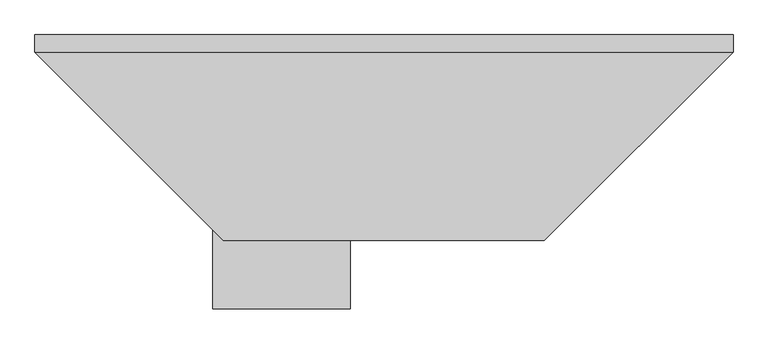
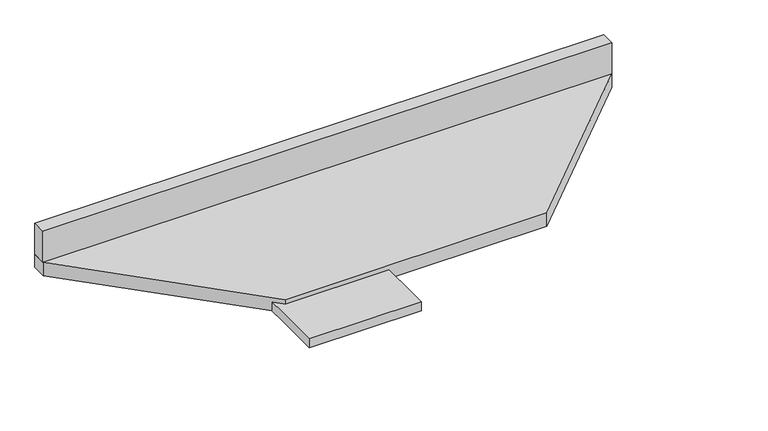
"""IFC4 building model written with IfcOpenShell, lengths in millimetres: proxy geometry, CT020 - Countertop, SS, No Opening - Angled : CT020 - Countertop, SS, No Opening - Angled."""

import ifcopenshell
import ifcopenshell.guid

model = None  # the IFC model being written
_history = None  # IfcOwnerHistory: only IFC2X3 demands one
_inside = {}  # id of a spatial element -> (the spatial element, [elements in it])
_under = {}  # id of a project, library or spatial element -> (it, [spatial elements below it])
_declared = {}  # id of a project -> (the project, [libraries it declares])
_typed = {}  # id of a type object -> (the type object, [elements of that type])
_made_of = {}  # id of a material, layer set ... -> (it, [elements and type objects made of it])


def new_model(schema):
    """Start an empty IFC model of exactly this schema.

    Asked for "IFC4X3", IfcOpenShell would pick the latest addendum, in which some entities
    have other attributes; the version numbers below select the first issue.
    IFC2X3 requires an IfcOwnerHistory on every rooted entity: one is made here for all.
    """
    global model, _history
    if schema == "IFC4X3":
        model = ifcopenshell.file(schema_version=(4, 3, 0, 0))
    else:
        model = ifcopenshell.file(schema=schema)
    _inside.clear()
    _under.clear()
    _declared.clear()
    _typed.clear()
    _made_of.clear()
    _history = None
    if model.schema == "IFC2X3":
        org = make("IfcOrganization", Name="unknown")
        user = make(
            "IfcPersonAndOrganization",
            ThePerson=make("IfcPerson", FamilyName="unknown"),
            TheOrganization=org,
        )
        app = make(
            "IfcApplication",
            ApplicationDeveloper=org,
            Version="unknown",
            ApplicationFullName="unknown",
            ApplicationIdentifier="unknown",
        )
        _history = make(
            "IfcOwnerHistory",
            OwningUser=user,
            OwningApplication=app,
            ChangeAction="ADDED",
            CreationDate=0,
        )
    return model


def make(cls, **values):
    """One entity of the class cls with the attributes given. An attribute that is None is left unset."""
    return model.create_entity(
        cls, **{name: value for name, value in values.items() if value is not None}
    )


def rooted(cls, **values):
    """An entity with a GlobalId (a new one), such as an element, a storey or a relation."""
    return make(cls, GlobalId=ifcopenshell.guid.new(), OwnerHistory=_history, **values)


def si_unit(unit_type, name, prefix=None):
    """IfcSIUnit, for example si_unit("LENGTHUNIT", "METRE", prefix="MILLI")."""
    return make("IfcSIUnit", UnitType=unit_type, Prefix=prefix, Name=name)


def assignment(units):
    """IfcUnitAssignment: the units of a project."""
    return None if units is None else make("IfcUnitAssignment", Units=units)


def point(xyz):
    """IfcCartesianPoint."""
    return None if xyz is None else make("IfcCartesianPoint", Coordinates=xyz)


def direction(xyz):
    """IfcDirection."""
    return None if xyz is None else make("IfcDirection", DirectionRatios=xyz)


def frame(location, z_axis=None, x_axis=None):
    """IfcAxis2Placement3D, a coordinate frame: its origin and axes. An axis left out is left unset."""
    return make(
        "IfcAxis2Placement3D",
        Location=point(location),
        Axis=direction(z_axis),
        RefDirection=direction(x_axis),
    )


def origin():
    """The frame at (0, 0, 0) with its axes left unset."""
    return frame((0.0, 0.0, 0.0))


def place(relative_to, where):
    """IfcLocalPlacement: puts the frame where relative to a parent placement (None: the world)."""
    return make(
        "IfcLocalPlacement", PlacementRelTo=relative_to, RelativePlacement=where
    )


def context(
    kind, dimensions, precision=None, world=None, true_north=None, identifier=None
):
    """IfcGeometricRepresentationContext, for example the 3D "Model" context."""
    return make(
        "IfcGeometricRepresentationContext",
        ContextIdentifier=identifier,
        ContextType=kind,
        CoordinateSpaceDimension=dimensions,
        Precision=precision,
        WorldCoordinateSystem=world,
        TrueNorth=true_north,
    )


def project(units=None, contexts=None):
    """IfcProject with its units and contexts."""
    return rooted(
        "IfcProject",
        Name="project",
        RepresentationContexts=contexts,
        UnitsInContext=assignment(units),
    )


def spatial(cls, under=None, at=None, **own):
    """A site, building, storey or space (cls), placed at a placement, below another one or the project."""
    s = rooted(cls, ObjectPlacement=at, **own)
    if under is not None:
        _under.setdefault(under.id(), (under, []))[1].append(s)
    return s


def polyline(points):
    """IfcPolyline through the points."""
    return make("IfcPolyline", Points=[point(p) for p in points])


def outline(outer, holes=None, kind="AREA"):
    """IfcArbitraryClosedProfileDef: a profile drawn as a closed curve; with holes, ...WithVoids."""
    if holes is None:
        return make("IfcArbitraryClosedProfileDef", ProfileType=kind, OuterCurve=outer)
    return make(
        "IfcArbitraryProfileDefWithVoids",
        ProfileType=kind,
        OuterCurve=outer,
        InnerCurves=holes,
    )


def extrude(swept, where, along, depth):
    """IfcExtrudedAreaSolid: the profile swept, set in the frame where, extruded along a direction by depth."""
    return make(
        "IfcExtrudedAreaSolid",
        SweptArea=swept,
        Position=where,
        ExtrudedDirection=direction(along),
        Depth=depth,
    )


def shape(context_of_items, identifier, shape_type, items):
    """IfcShapeRepresentation: the items that make up one representation, for example the "Body"."""
    return make(
        "IfcShapeRepresentation",
        ContextOfItems=context_of_items,
        RepresentationIdentifier=identifier,
        RepresentationType=shape_type,
        Items=items,
    )


def source(mapping_origin, context_of_items, identifier, shape_type, items):
    """IfcRepresentationMap: a shape defined once, which mapped items show again and again."""
    return make(
        "IfcRepresentationMap",
        MappingOrigin=mapping_origin,
        MappedRepresentation=shape(context_of_items, identifier, shape_type, items),
    )


def transform(
    local_origin,
    x_axis=None,
    y_axis=None,
    z_axis=None,
    scale=None,
    scale2=None,
    scale3=None,
    uniform=True,
):
    """IfcCartesianTransformationOperator3D, or its non-uniform kind. x_axis, y_axis, z_axis: its Axis1, 2, 3."""
    if uniform:
        return make(
            "IfcCartesianTransformationOperator3D",
            Axis1=direction(x_axis),
            Axis2=direction(y_axis),
            LocalOrigin=point(local_origin),
            Scale=scale,
            Axis3=direction(z_axis),
        )
    return make(
        "IfcCartesianTransformationOperator3DnonUniform",
        Axis1=direction(x_axis),
        Axis2=direction(y_axis),
        LocalOrigin=point(local_origin),
        Scale=scale,
        Axis3=direction(z_axis),
        Scale2=scale2,
        Scale3=scale3,
    )


def mapped(mapping_source, mapping_target):
    """IfcMappedItem: shows the shape of a source again, moved by a transform."""
    return make(
        "IfcMappedItem", MappingSource=mapping_source, MappingTarget=mapping_target
    )


def made_of(thing, what):
    """Note that an element or type object is made of a material, layer set ...; save() writes the relation."""
    if what is not None:
        _made_of.setdefault(what.id(), (what, []))[1].append(thing)
    return thing


def element(
    cls,
    number,
    at=None,
    inside=None,
    cuts=None,
    type_object=None,
    material=None,
    context=None,
    identifier="Body",
    shape_type=None,
    held_by="IfcProductDefinitionShape",
    body=None,
    shapes=None,
    **own,
):
    """One element of the class cls, such as IfcWall. Its Tag is "e" and its number.

    at: its placement. inside: the storey or other place that contains it. cuts: it is an
    opening in that element (IfcRelVoidsElement). A single representation is given by context,
    identifier, shape_type and body (its items); several are given by shapes. held_by: the class
    of the entity that holds the representations. save() writes the other relations.
    """
    e = rooted(cls, Tag="e%d" % number, ObjectPlacement=at, **own)
    if body is not None:
        shapes = [shape(context, identifier, shape_type, body)]
    if shapes is not None:
        e.Representation = make(held_by, Representations=shapes)
    if inside is not None:
        _inside.setdefault(inside.id(), (inside, []))[1].append(e)
    if cuts is not None:
        rooted(
            "IfcRelVoidsElement", RelatingBuildingElement=cuts, RelatedOpeningElement=e
        )
    if type_object is not None:
        _typed.setdefault(type_object.id(), (type_object, []))[1].append(e)
    return made_of(e, material)


def aggregate(whole, parts):
    """IfcRelAggregates: a whole, such as a stair, and the parts it consists of."""
    return rooted("IfcRelAggregates", RelatingObject=whole, RelatedObjects=parts)


def save(model, path):
    """Write the relations noted so far, then the file.

    IfcRelAggregates (storeys below a building ...), IfcRelContainedInSpatialStructure (elements
    in a storey), IfcRelDefinesByType, IfcRelAssociatesMaterial and IfcRelDeclares: one each for
    every whole, place, type object, material and project.
    """
    for whole, parts in _under.values():
        aggregate(whole, parts)
    for where, things in _inside.values():
        rooted(
            "IfcRelContainedInSpatialStructure",
            RelatedElements=things,
            RelatingStructure=where,
        )
    for kind, things in _typed.values():
        rooted("IfcRelDefinesByType", RelatedObjects=things, RelatingType=kind)
    for what, things in _made_of.values():
        rooted("IfcRelAssociatesMaterial", RelatedObjects=things, RelatingMaterial=what)
    for by, libraries in _declared.values():
        rooted("IfcRelDeclares", RelatingContext=by, RelatedDefinitions=libraries)
    model.write(path)


def specialty_equipment_e7a2204c(model_context):
    return source(origin(), model_context, "Body", "SweptSolid", [
        extrude(outline(polyline([(-547.6510783, 266.7), (-547.6510783, 304.8), (1002.6430003, 304.8), (1002.6430003, 266.7), (-547.6510783, 266.7)])), frame((0.0, 0.0, 876.3), z_axis=(0.0, 0.0, 1.0), x_axis=(1.0, 0.0, 0.0)), (0.0, 0.0, 1.0), 88.9),
        extrude(outline(polyline([(1002.6430003, 304.8), (1002.6430003, 266.6686289), (583.5743714, -152.4), (-129.1499366, -152.4), (-547.6510783, 266.1011418), (-547.6510783, 304.8), (1002.6430003, 304.8)])), frame((0.0, 0.0, 838.2), z_axis=(0.0, 0.0, 1.0), x_axis=(1.0, 0.0, 0.0)), (0.0, 0.0, 1.0), 38.1),
        extrude(outline(polyline([(-152.4, 304.8), (152.4, 304.8), (152.4, -304.8), (-152.4, -304.8), (-152.4, 0.0), (-152.4, 304.8)])), frame((0.0, 0.0, 838.2), z_axis=(0.0, 0.0, 1.0), x_axis=(1.0, 0.0, 0.0)), (0.0, 0.0, 1.0), 25.4),
    ])


if __name__ == "__main__":
    model = new_model("IFC4")
    model_context = context("Model", 3, world=origin())
    ifc_project = project(units=[si_unit("LENGTHUNIT", "METRE", prefix="MILLI")], contexts=[model_context])
    site = spatial("IfcSite", under=ifc_project)
    building = spatial("IfcBuilding", under=site)
    placement = place(None, origin())
    specialty_equipment_shape = specialty_equipment_e7a2204c(model_context)
    element("IfcBuildingElementProxy", 1, Name="CT020 - Countertop, SS, No Opening - Angled : CT020 - Countertop, SS, No Opening - Angled", ObjectType="CT020 - Countertop, SS, No Opening - Angled : CT020 - Countertop, SS, No Opening - Angled", at=placement, inside=building, context=model_context, shape_type="MappedRepresentation", body=[
        mapped(specialty_equipment_shape, transform((0.0, 0.0, 0.0), x_axis=(1.0, 0.0, 0.0), y_axis=(0.0, 1.0, 0.0), z_axis=(0.0, 0.0, 1.0))),
    ])
    save(model, "model.ifc")

# Revit data of these elements
# Type "CT020 - Countertop, SS, No Opening - Angled : CT020 - Countertop, SS, No Opening - Angled"
#   Watts2 = "0"
#   Watts1 = "0"
#   Unit_Issue = "LF"
#   UTIL_6_Misc = "-"
#   UTIL_5_NonMedGas = "-"
#   UTIL_4_MiscGas = "-"
#   UTIL_3_MedGas = "-"
#   UTIL_2_Elec = "-"
#   UTIL_1_WaterDrain = "-"
#   Nomenclature = "Countertop, Solid Surface, Angled"
#   NSN = ""
#   Location [instance default] = ""
#   JSN = "CT020"
#   Fund_Source_VA = "-"
#   Fund_Source_Navy = "-"
#   Fund_Source_Army = "-"
#   Fund_Source_AF = "-"
#   ELEC_Volts2 = "0"
#   ELEC_Volts1 = "0"
#   ELEC_Phase2 = "0"
#   ELEC_Phase1 = "0"
#   ELEC_HertzSwitch = "0"
#   ELEC_HertzDependent = "0"
#   ELEC_Hertz = "0"
#   ELEC_Amps2 = "0"
#   ELEC_Amps1 = "0"
#   DetailDescription = ""
#   CAT_VA = "A"
#   CAT_Navy = "A"
#   CAT_IHS = "-"
#   CAT_Army = "A"
#   CAT_AF = "A"
#   BTUperhour = "0"
#   Weight_IP = 14
#   DIM_Width_IP = 1' - 0"
#   DIM_Height_IP = 0' - 1"
#   DIM_Depth_IP = 2' - 0"
#   CustomLength [instance default] = 4' - 0"
#   Assembly Code = ""
# Element 1 (IfcBuildingElementProxy, "CT020 - Countertop, SS, No Opening - Angled : CT020 - Countertop, SS, No Opening - Angled")
#   Materials on its faces: "CounterTopFinish", "EquipSpace"
# Materials
#   "CounterTopFinish": class "Unassigned", colour RGB 139 121 96, transparency 0
#   "EquipSpace": class "Unassigned", colour RGB 221 217 195, transparency 0.5
